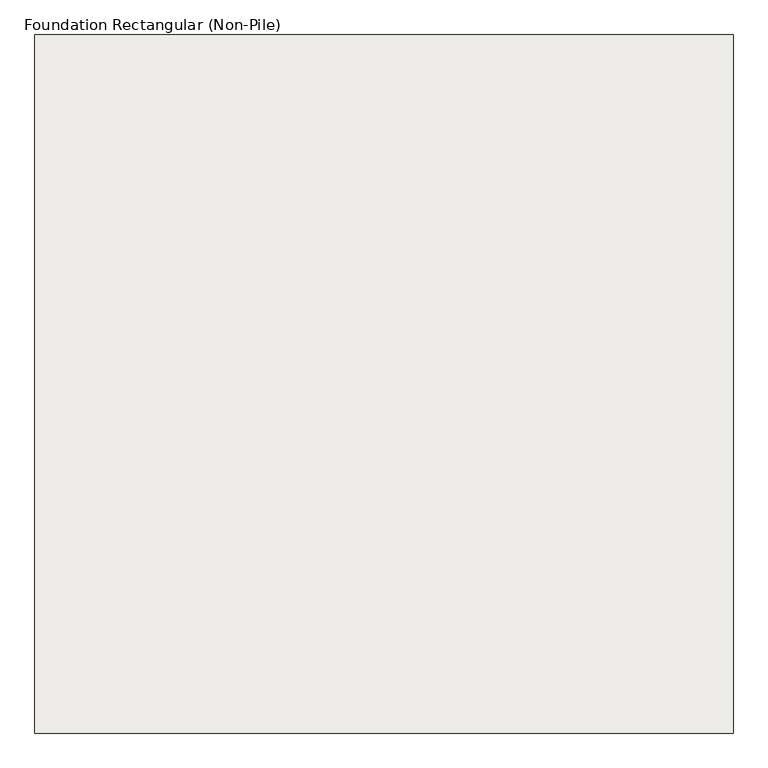
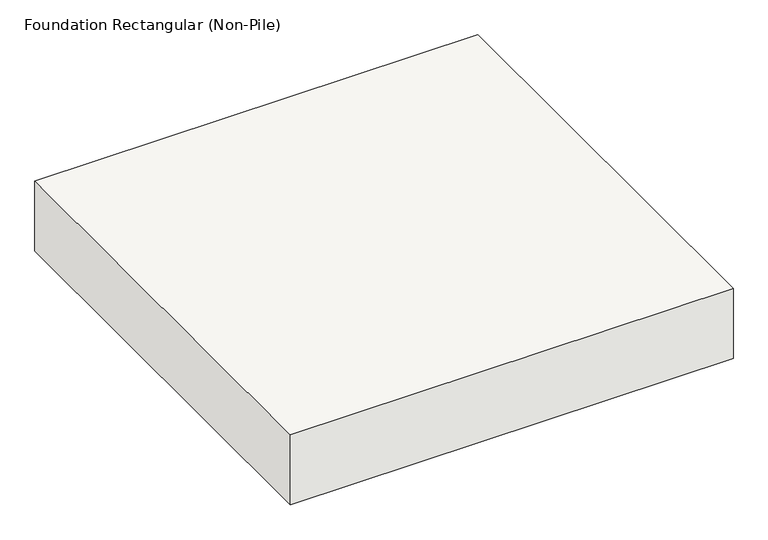
"""IFC4 building model written with IfcOpenShell, lengths in millimetres: slab geometry, Foundation Rectangular (Non-Pile) : H_SF_AR S18_Ret Fdn_F2 3000x3000x500."""

from ifc_helpers import new_model, si_unit, frame, origin, place, context, project, spatial, polyline, outline, extrude, source, transform, mapped, element, save


def foundation_rectangular_non_pile_a43cc813(model_context):
    return source(origin(), model_context, "Body", "SweptSolid", [
        extrude(outline(polyline([(1500.0, 1500.0), (1500.0, -1500.0), (-1500.0, -1500.0), (-1500.0, 1500.0), (1500.0, 1500.0)])), frame((0.0, 0.0, -500.0), z_axis=(0.0, 0.0, 1.0), x_axis=(1.0, 0.0, 0.0)), (0.0, 0.0, 1.0), 500.0),
    ])


if __name__ == "__main__":
    model = new_model("IFC4")
    model_context = context("Model", 3, world=origin())
    ifc_project = project(units=[si_unit("LENGTHUNIT", "METRE", prefix="MILLI")], contexts=[model_context])
    site = spatial("IfcSite", under=ifc_project)
    building = spatial("IfcBuilding", under=site)
    placement = place(None, origin())
    foundation_rectangular_non_pile_shape = foundation_rectangular_non_pile_a43cc813(model_context)
    element("IfcSlab", 1, ObjectType="Foundation Rectangular (Non-Pile) : H_SF_AR S18_Ret Fdn_F2 3000x3000x500", at=placement, inside=building, context=model_context, shape_type="MappedRepresentation", body=[
        mapped(foundation_rectangular_non_pile_shape, transform((0.0, 0.0, 0.0), x_axis=(1.0, 0.0, 0.0), y_axis=(0.0, 1.0, 0.0), z_axis=(0.0, 0.0, 1.0))),
    ])
    save(model, "model.ifc")

# Revit data of these elements
# Type "Foundation Rectangular (Non-Pile) : H_SF_AR S18_Ret Fdn_F2 3000x3000x500"
#   Type Comments = "UG"
#   Type Mark = "F2"
#   Top bar = "D25@300"
#   Description = "UG Shallow Foundation"
#   Bottom bar = "D20@300"
#   H_Rebar Ratio = 0.12
#   Width = 3000 mm
#   Length = 3000 mm
#   Foundation Thickness = 500 mm
#   Structural Material [instance default] = none
#   Assembly Code = ""
# Element 1 (IfcSlab, "Foundation Rectangular (Non-Pile) : H_SF_AR S18_Ret Fdn_F2 3000x3000x500")
#   Materials on its faces: "00_Concrete_Reinf. Conc."
# Materials
#   "00_Concrete_Reinf. Conc.": class "Concrete", colour RGB 176 176 176, transparency 0, Description = "Reinf. Conc.", Cost = 0, Image = Concrete.Cast-In-Place.Flat.Polished.Grey.jpg
